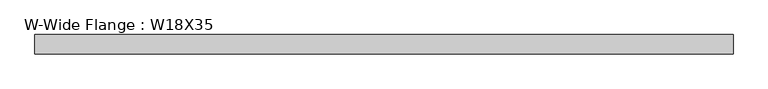
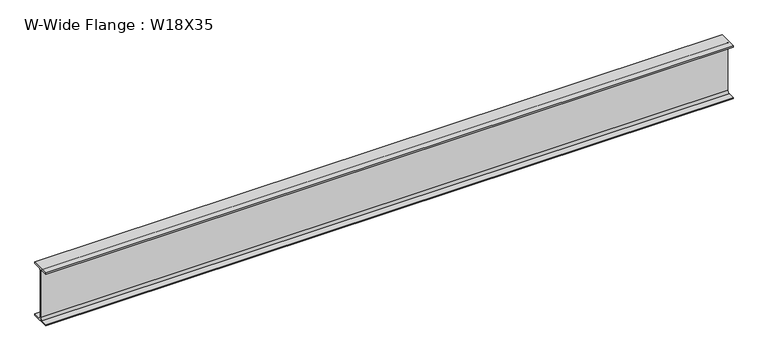
"""IFC4 building model written with IfcOpenShell, lengths in millimetres: beam geometry, W-Wide Flange : W18X35."""

from ifc_helpers import new_model, si_unit, point, frame, frame_2d, origin, place, context, project, spatial, polyline, circle_curve, trimmed, segment, composite_curve, outline, extrude, source, transform, mapped, element, save


def w_wide_flange_w18x35_2f8c58f8(model_context):
    return source(origin(), model_context, "Body", "SweptSolid", [
        extrude(outline(composite_curve([segment(polyline([(76.2, -213.995), (76.2, -224.79), (-76.2, -224.79), (-76.2, -213.995), (-21.59, -213.995)]), True, "CONTINUOUS"), segment(trimmed(circle_curve(frame_2d((-21.59, -196.215)), 17.78), [point((-21.59, -213.995))], [point((-3.81, -196.215))], True, "CARTESIAN"), True, "CONTINUOUS"), segment(polyline([(-3.81, -196.215), (-3.81, 196.215)]), True, "CONTINUOUS"), segment(trimmed(circle_curve(frame_2d((-21.59, 196.215)), 17.78), [point((-3.81, 196.215))], [point((-21.59, 213.995))], True, "CARTESIAN"), True, "CONTINUOUS"), segment(polyline([(-21.59, 213.995), (-76.2, 213.995), (-76.2, 224.79), (76.2, 224.79), (76.2, 213.995), (21.59, 213.995)]), True, "CONTINUOUS"), segment(trimmed(circle_curve(frame_2d((21.59, 196.215)), 17.78), [point((21.59, 213.995))], [point((3.81, 196.215))], True, "CARTESIAN"), True, "CONTINUOUS"), segment(polyline([(3.81, 196.215), (3.81, -196.215)]), True, "CONTINUOUS"), segment(trimmed(circle_curve(frame_2d((21.59, -196.215)), 17.78), [point((3.81, -196.215))], [point((21.59, -213.995))], True, "CARTESIAN"), True, "CONTINUOUS"), segment(polyline([(21.59, -213.995), (76.2, -213.995)]), True, "CONTINUOUS")], self_intersect=False)), frame((-2755.9, 0.0, 0.0), z_axis=(1.0, 0.0, 0.0), x_axis=(0.0, 1.0, 0.0)), (0.0, 0.0, 1.0), 5511.8),
    ])


if __name__ == "__main__":
    model = new_model("IFC4")
    model_context = context("Model", 3, world=origin())
    ifc_project = project(units=[si_unit("LENGTHUNIT", "METRE", prefix="MILLI")], contexts=[model_context])
    site = spatial("IfcSite", under=ifc_project)
    building = spatial("IfcBuilding", under=site)
    placement = place(None, origin())
    w_wide_flange_w18x35_shape = w_wide_flange_w18x35_2f8c58f8(model_context)
    element("IfcBeam", 1, ObjectType="W-Wide Flange : W18X35", at=placement, inside=building, context=model_context, shape_type="MappedRepresentation", body=[
        mapped(w_wide_flange_w18x35_shape, transform((0.0, 0.0, 0.0), x_axis=(1.0, 0.0, 0.0), y_axis=(0.0, 1.0, 0.0), z_axis=(0.0, 0.0, 1.0))),
    ])
    save(model, "model.ifc")

# Revit data of these elements
# Type "W-Wide Flange : W18X35"
#   Assembly Code = "B10"
#   W = 35
#   Length [instance default] = 5' - 0"
#   bf = 0' - 6"
#   d = 1' - 5.7"
#   k = 0' - 1 1/8"
#   k2 = 0' - 0.7"
#   tf = 0' - 0.425"
#   tw = 0' - 0.3"
#   A = 0.0715278 SF
#   Structural Material [instance default] = Steel ASTM A992
# Element 1 (IfcBeam, "W-Wide Flange : W18X35")
#   Materials on its faces: "Steel ASTM A992"
# Materials
#   "Steel ASTM A992": class "Metal", colour RGB 199 199 199, transparency 0, Description = "Structural steel 50ksi", Cost = 0
